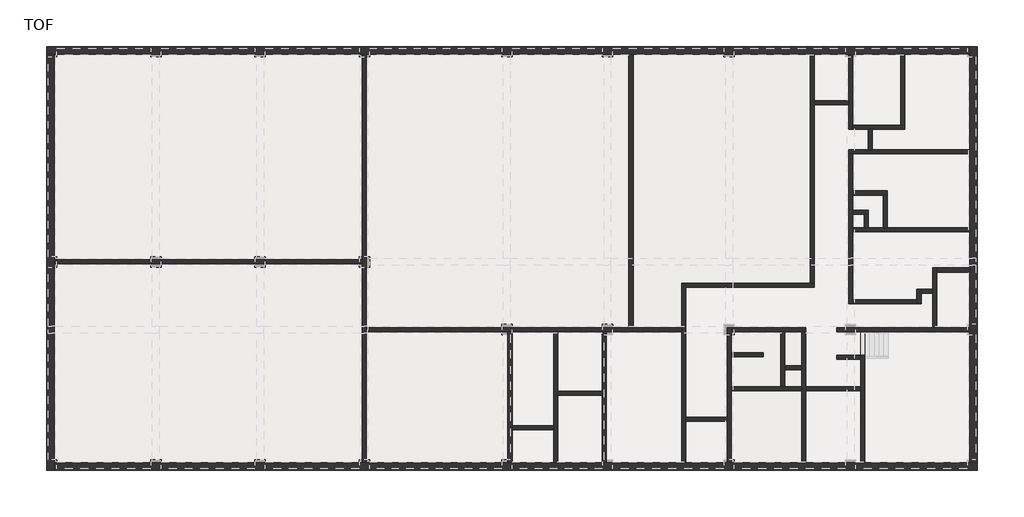
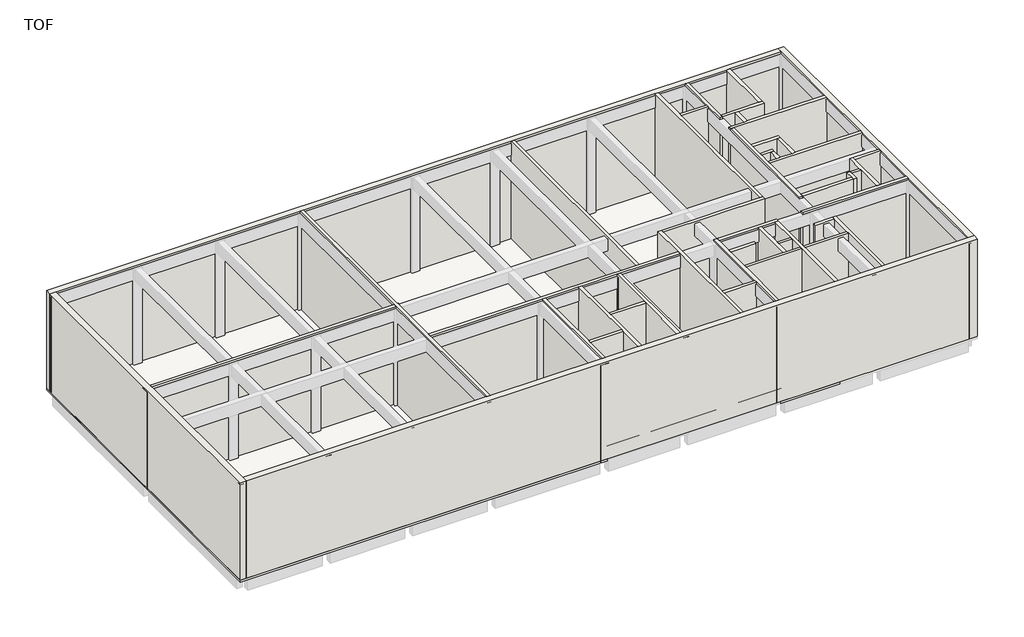
# One storey, part 1 of 3: 45 walls, 3 slabs.
"""IFC4 building model written with IfcOpenShell, lengths in millimetres."""

from ifc_helpers import new_model, si_unit, frame, origin, origin_with_axes, place, context, project, spatial, polyline, outline, extrude, faceted_brep, element, save

model = new_model("IFC4")

# Units and contexts
model_context = context("Model", 3, world=origin())
ifc_project = project(units=[si_unit("LENGTHUNIT", "METRE", prefix="MILLI")], contexts=[model_context])

# Site, building, storey
site = spatial("IfcSite", under=ifc_project)
building = spatial("IfcBuilding", under=site)
storey = spatial("IfcBuildingStorey", under=building, Name="TOF", Elevation=150.0)

# Slabs
placement = place(None, origin())
element("IfcSlab", 1, ObjectType="H_FL_AMF_RC Slab_T150", at=placement, inside=storey, context=model_context, shape_type="Brep", body=[
    faceted_brep([(-375.3, 24716.5208589, 0.0), (43724.7, 24716.5208589, 0.0), (43724.7, 10966.5208589, 0.0), (36324.7, 10966.5208589, 0.0), (36324.7, 8416.5208589, 0.0), (32224.7, 8416.5208589, 0.0), (31624.7, 8416.5208589, 0.0), (26424.7, 8416.5208589, 0.0), (25824.7, 8416.5208589, 0.0), (17924.7, 8416.5208589, 0.0), (17924.7, 12016.5208589, 0.0), (17924.7, 12316.5208589, 0.0), (17624.7, 12316.5208589, 0.0), (12224.7, 12316.5208589, 0.0), (11624.7, 12316.5208589, 0.0), (6224.7, 12316.5208589, 0.0), (5624.7, 12316.5208589, 0.0), (224.7, 12316.5208589, 0.0), (-375.3, 12316.5208589, 0.0), (-375.3, 24716.5208589, 150.0), (-375.3, 24116.5208589, 150.0), (-375.3, 12616.5208589, 150.0), (-375.3, 12316.5208589, 150.0), (224.7, 12316.5208589, 150.0), (5624.7, 12316.5208589, 150.0), (6224.7, 12316.5208589, 150.0), (11624.7, 12316.5208589, 150.0), (12224.7, 12316.5208589, 150.0), (17624.7, 12316.5208589, 150.0), (17924.7, 12316.5208589, 150.0), (17924.7, 12016.5208589, 150.0), (17924.7, 8416.5208589, 150.0), (25824.7, 8416.5208589, 150.0), (26424.7, 8416.5208589, 150.0), (31624.7, 8416.5208589, 150.0), (32224.7, 8416.5208589, 150.0), (36324.7, 8416.5208589, 150.0), (36324.7, 10966.5208589, 150.0), (43724.7, 10966.5208589, 150.0), (43724.7, 24716.5208589, 150.0), (39224.7, 24716.5208589, 150.0), (38624.7, 24716.5208589, 150.0), (32224.7, 24716.5208589, 150.0), (31624.7, 24716.5208589, 150.0), (26424.7, 24716.5208589, 150.0), (25824.7, 24716.5208589, 150.0), (18224.7, 24716.5208589, 150.0), (17624.7, 24716.5208589, 150.0), (12224.7, 24716.5208589, 150.0), (11624.7, 24716.5208589, 150.0), (6224.7, 24716.5208589, 150.0), (5624.7, 24716.5208589, 150.0), (224.7, 24716.5208589, 150.0)], [[[0, 1, 2, 3, 4, 5, 6, 7, 8, 9, 10, 11, 12, 13, 14, 15, 16, 17, 18]], [[19, 20, 21, 22, 23, 24, 25, 26, 27, 28, 29, 30, 31, 32, 33, 34, 35, 36, 37, 38, 39, 40, 41, 42, 43, 44, 45, 46, 47, 48, 49, 50, 51, 52]], [[0, 18, 22, 21, 20, 19]], [[1, 0, 19, 52, 51, 50, 49, 48, 47, 46, 45, 44, 43, 42, 41, 40, 39]], [[2, 1, 39, 38]], [[3, 2, 38, 37]], [[4, 3, 37, 36]], [[9, 8, 7, 6, 5, 4, 36, 35, 34, 33, 32, 31]], [[11, 10, 9, 31, 30, 29]], [[18, 17, 16, 15, 14, 13, 12, 11, 29, 28, 27, 26, 25, 24, 23, 22]]]),
])
element("IfcSlab", 2, ObjectType="H_FL_AMF_RC Slab_T150", at=placement, inside=storey, context=model_context, shape_type="SweptSolid", body=[
    extrude(outline(polyline([(17924.7, 12316.5208589), (17924.7, 8416.5208589), (26307.7, 8416.5208589), (26307.7, 316.5208589), (-375.3, 316.5208589), (-375.3, 12316.5208589), (17924.7, 12316.5208589)])), origin_with_axes(), (0.0, 0.0, 1.0), 150.0),
])
element("IfcSlab", 3, ObjectType="H_FL_AMF_RC Slab_T150", at=placement, inside=storey, context=model_context, shape_type="SweptSolid", body=[
    extrude(outline(polyline([(38924.7, 316.5208589), (38924.7, 8416.5208589), (43224.7, 8416.5208589), (43224.7, 316.5208589), (38924.7, 316.5208589)])), origin_with_axes(), (0.0, 0.0, 1.0), 150.0),
])

# Walls
element("IfcWall", 4, ObjectType="H_WA_AMW_Brick Wall_Ext (0.5B_50_1.0B / Emulsion)", at=placement, inside=storey, context=model_context, shape_type="Brep", body=[
    faceted_brep([(-375.3, 24286.5208589, 150.0), (54.7, 24286.5208589, 150.0), (17807.7, 24286.5208589, 150.0), (18041.7, 24286.5208589, 150.0), (33157.7, 24286.5208589, 150.0), (33391.7, 24286.5208589, 150.0), (43607.7, 24286.5208589, 150.0), (43841.7, 24286.5208589, 150.0), (52794.7, 24286.5208589, 150.0), (52794.7, 24286.5208589, 7650.0), (49041.7, 24286.5208589, 7650.0), (48807.7, 24286.5208589, 7650.0), (46041.7, 24286.5208589, 7650.0), (45807.7, 24286.5208589, 7650.0), (43841.7, 24286.5208589, 7650.0), (43607.7, 24286.5208589, 7650.0), (33391.7, 24286.5208589, 7650.0), (33157.7, 24286.5208589, 7650.0), (18041.7, 24286.5208589, 7650.0), (17807.7, 24286.5208589, 7650.0), (54.7, 24286.5208589, 7650.0), (-375.3, 24286.5208589, 7650.0), (-375.3, 24716.5208589, 150.0), (-375.3, 24716.5208589, 7650.0), (52794.7, 24716.5208589, 7650.0), (52794.7, 24716.5208589, 150.0)], [[[0, 1, 2, 3, 4, 5, 6, 7, 8, 9, 10, 11, 12, 13, 14, 15, 16, 17, 18, 19, 20, 21]], [[22, 23, 24, 25]], [[8, 7, 6, 5, 4, 3, 2, 1, 0, 22, 25]], [[21, 20, 19, 18, 17, 16, 15, 14, 13, 12, 11, 10, 9, 24, 23]], [[0, 21, 23, 22]], [[9, 8, 25, 24]]]),
])
element("IfcWall", 5, ObjectType="H_WA_AMW_Brick Wall_Ext (0.5B_50_1.0B / Emulsion)", at=placement, inside=storey, context=model_context, shape_type="Brep", body=[
    faceted_brep([(54.7, 316.5208589, 150.0), (54.7, 746.5208589, 150.0), (54.7, 12199.5208589, 150.0), (54.7, 12433.5208589, 150.0), (54.7, 24286.5208589, 150.0), (54.7, 24286.5208589, 7650.0), (54.7, 12433.5208589, 7650.0), (54.7, 12199.5208589, 7650.0), (54.7, 746.5208589, 7650.0), (54.7, 316.5208589, 7650.0), (-375.3, 316.5208589, 150.0), (-375.3, 316.5208589, 7650.0), (-375.3, 24286.5208589, 7650.0), (-375.3, 24286.5208589, 150.0)], [[[0, 1, 2, 3, 4, 5, 6, 7, 8, 9]], [[10, 11, 12, 13]], [[4, 3, 2, 1, 0, 10, 13]], [[9, 8, 7, 6, 5, 12, 11]], [[0, 9, 11, 10]], [[5, 4, 13, 12]]]),
])
element("IfcWall", 6, ObjectType="H_WA_AMW_Brick Wall_Ext (0.5B_50_1.0B / Emulsion)", at=placement, inside=storey, context=model_context, shape_type="Brep", body=[
    faceted_brep([(53224.7, 746.5208589, 150.0), (52794.7, 746.5208589, 150.0), (46741.7, 746.5208589, 150.0), (46507.7, 746.5208589, 150.0), (43341.7, 746.5208589, 150.0), (43107.7, 746.5208589, 150.0), (39041.7, 746.5208589, 150.0), (38807.7, 746.5208589, 150.0), (26424.7, 746.5208589, 150.0), (26190.7, 746.5208589, 150.0), (18041.7, 746.5208589, 150.0), (17807.7, 746.5208589, 150.0), (54.7, 746.5208589, 150.0), (54.7, 746.5208589, 7650.0), (17807.7, 746.5208589, 7650.0), (18041.7, 746.5208589, 7650.0), (26190.7, 746.5208589, 7650.0), (26424.7, 746.5208589, 7650.0), (28824.7, 746.5208589, 7650.0), (29058.7, 746.5208589, 7650.0), (31624.7, 746.5208589, 7650.0), (31858.7, 746.5208589, 7650.0), (36207.7, 746.5208589, 7650.0), (36441.7, 746.5208589, 7650.0), (38807.7, 746.5208589, 7650.0), (39041.7, 746.5208589, 7650.0), (43107.7, 746.5208589, 7650.0), (43341.7, 746.5208589, 7650.0), (46507.7, 746.5208589, 7650.0), (46741.7, 746.5208589, 7650.0), (52794.7, 746.5208589, 7650.0), (53224.7, 746.5208589, 7650.0), (53224.7, 316.5208589, 150.0), (53224.7, 316.5208589, 7650.0), (54.7, 316.5208589, 7650.0), (54.7, 316.5208589, 150.0)], [[[0, 1, 2, 3, 4, 5, 6, 7, 8, 9, 10, 11, 12, 13, 14, 15, 16, 17, 18, 19, 20, 21, 22, 23, 24, 25, 26, 27, 28, 29, 30, 31]], [[32, 33, 34, 35]], [[12, 11, 10, 9, 8, 7, 6, 5, 4, 3, 2, 1, 0, 32, 35]], [[31, 30, 29, 28, 27, 26, 25, 24, 23, 22, 21, 20, 19, 18, 17, 16, 15, 14, 13, 34, 33]], [[0, 31, 33, 32]], [[13, 12, 35, 34]]]),
])
element("IfcWall", 7, ObjectType="H_WA_AMW_Brick Wall_Ext (0.5B_50_1.0B / Emulsion)", at=placement, inside=storey, context=model_context, shape_type="Brep", body=[
    faceted_brep([(52794.7, 24716.5208589, 150.0), (52794.7, 24286.5208589, 150.0), (52794.7, 8533.5208589, 150.0), (52794.7, 8299.5208589, 150.0), (52794.7, 746.5208589, 150.0), (52794.7, 746.5208589, 7650.0), (52794.7, 8299.5208589, 7650.0), (52794.7, 8533.5208589, 7650.0), (52794.7, 11733.5208589, 7650.0), (52794.7, 11967.5208589, 7650.0), (52794.7, 14049.5208589, 7650.0), (52794.7, 14283.5208589, 7650.0), (52794.7, 18549.5208589, 7650.0), (52794.7, 18783.5208589, 7650.0), (52794.7, 24286.5208589, 7650.0), (52794.7, 24716.5208589, 7650.0), (53224.7, 24716.5208589, 150.0), (53224.7, 24716.5208589, 7650.0), (53224.7, 746.5208589, 7650.0), (53224.7, 746.5208589, 150.0)], [[[0, 1, 2, 3, 4, 5, 6, 7, 8, 9, 10, 11, 12, 13, 14, 15]], [[16, 17, 18, 19]], [[4, 3, 2, 1, 0, 16, 19]], [[15, 14, 13, 12, 11, 10, 9, 8, 7, 6, 5, 18, 17]], [[0, 15, 17, 16]], [[5, 4, 19, 18]]]),
])
element("IfcWall", 8, ObjectType="H_WA_AMW_Block Wall_Int_T200 (Both Plaster_Emulsion)", at=placement, inside=storey, context=model_context, shape_type="SweptSolid", body=[
    extrude(outline(polyline([(17807.7, 12199.5208589), (54.7, 12199.5208589), (54.7, 12433.5208589), (17807.7, 12433.5208589), (17807.7, 12199.5208589)])), frame((0.0, 0.0, 150.0), z_axis=(0.0, 0.0, 1.0), x_axis=(1.0, 0.0, 0.0)), (0.0, 0.0, 1.0), 7500.0),
])
element("IfcWall", 9, ObjectType="H_WA_AMW_Block Wall_Int_T200 (Both Plaster_Emulsion)", at=placement, inside=storey, context=model_context, shape_type="Brep", body=[
    faceted_brep([(17807.7, 24286.5208589, 150.0), (17807.7, 12433.5208589, 150.0), (17807.7, 12199.5208589, 150.0), (17807.7, 746.5208589, 150.0), (17807.7, 746.5208589, 7650.0), (17807.7, 12199.5208589, 7650.0), (17807.7, 12433.5208589, 7650.0), (17807.7, 24286.5208589, 7650.0), (18041.7, 24286.5208589, 150.0), (18041.7, 24286.5208589, 7650.0), (18041.7, 8533.5208589, 7650.0), (18041.7, 8299.5208589, 7650.0), (18041.7, 746.5208589, 7650.0), (18041.7, 746.5208589, 150.0), (18041.7, 8299.5208589, 150.0), (18041.7, 8533.5208589, 150.0)], [[[0, 1, 2, 3, 4, 5, 6, 7]], [[8, 9, 10, 11, 12, 13, 14, 15]], [[3, 2, 1, 0, 8, 15, 14, 13]], [[7, 6, 5, 4, 12, 11, 10, 9]], [[0, 7, 9, 8]], [[4, 3, 13, 12]]]),
])
element("IfcWall", 10, ObjectType="H_WA_AMW_Block Wall_Int_T200 (Both Plaster_Emulsion)", at=placement, inside=storey, context=model_context, shape_type="SweptSolid", body=[
    extrude(outline(polyline([(33157.7, 8533.5208589), (33157.7, 24286.5208589), (33391.7, 24286.5208589), (33391.7, 8533.5208589), (33157.7, 8533.5208589)])), frame((0.0, 0.0, 150.0), z_axis=(0.0, 0.0, 1.0), x_axis=(1.0, 0.0, 0.0)), (0.0, 0.0, 1.0), 7500.0),
])
element("IfcWall", 11, ObjectType="H_WA_AMW_Block Wall_Int_T200 (Both Plaster_Emulsion)", at=placement, inside=storey, context=model_context, shape_type="Brep", body=[
    faceted_brep([(18041.7, 8299.5208589, 150.0), (26190.7, 8299.5208589, 150.0), (26424.7, 8299.5208589, 150.0), (36207.7, 8299.5208589, 150.0), (36207.7, 8299.5208589, 7650.0), (31858.7, 8299.5208589, 7650.0), (31624.7, 8299.5208589, 7650.0), (29058.7, 8299.5208589, 7650.0), (28824.7, 8299.5208589, 7650.0), (26424.7, 8299.5208589, 7650.0), (26190.7, 8299.5208589, 7650.0), (18041.7, 8299.5208589, 7650.0), (18041.7, 8533.5208589, 150.0), (18041.7, 8533.5208589, 7650.0), (33157.7, 8533.5208589, 7650.0), (33391.7, 8533.5208589, 7650.0), (36207.7, 8533.5208589, 7650.0), (36207.7, 8533.5208589, 150.0), (33391.7, 8533.5208589, 150.0), (33157.7, 8533.5208589, 150.0)], [[[0, 1, 2, 3, 4, 5, 6, 7, 8, 9, 10, 11]], [[12, 13, 14, 15, 16, 17, 18, 19]], [[3, 2, 1, 0, 12, 19, 18, 17]], [[11, 10, 9, 8, 7, 6, 5, 4, 16, 15, 14, 13]], [[0, 11, 13, 12]], [[4, 3, 17, 16]]]),
])
element("IfcWall", 12, ObjectType="H_WA_AMW_Block Wall_Int_T200 (Both Plaster_Emulsion)", at=placement, inside=storey, context=model_context, shape_type="Brep", body=[
    faceted_brep([(36207.7, 11083.5208589, 1150.0), (36207.7, 746.5208589, 1150.0), (36207.7, 746.5208589, 7650.0), (36207.7, 8299.5208589, 7650.0), (36207.7, 8533.5208589, 7650.0), (36207.7, 11083.5208589, 7650.0), (36441.7, 11083.5208589, 1150.0), (36441.7, 11083.5208589, 7650.0), (36441.7, 10849.5208589, 7650.0), (36441.7, 3380.5208589, 7650.0), (36441.7, 3146.5208589, 7650.0), (36441.7, 746.5208589, 7650.0), (36441.7, 746.5208589, 1150.0), (36441.7, 3146.5208589, 1150.0), (36441.7, 3380.5208589, 1150.0)], [[[0, 1, 2, 3, 4, 5]], [[6, 7, 8, 9, 10, 11, 12, 13, 14]], [[1, 0, 6, 14, 13, 12]], [[5, 4, 3, 2, 11, 10, 9, 8, 7]], [[2, 1, 12, 11]], [[0, 5, 7, 6]]]),
])
element("IfcWall", 13, ObjectType="H_WA_AMW_Block Wall_Int_T200 (Both Plaster_Emulsion)", at=placement, inside=storey, context=model_context, shape_type="Brep", body=[
    faceted_brep([(36441.7, 10849.5208589, 150.0), (43841.7, 10849.5208589, 150.0), (43841.7, 10849.5208589, 7650.0), (36441.7, 10849.5208589, 7650.0), (36441.7, 11083.5208589, 150.0), (36441.7, 11083.5208589, 1150.0), (36441.7, 11083.5208589, 7650.0), (43607.7, 11083.5208589, 7650.0), (43841.7, 11083.5208589, 7650.0), (43841.7, 11083.5208589, 150.0), (43607.7, 11083.5208589, 150.0)], [[[0, 1, 2, 3]], [[4, 5, 6, 7, 8, 9, 10]], [[1, 0, 4, 10, 9]], [[3, 2, 8, 7, 6]], [[0, 3, 6, 5, 4]], [[2, 1, 9, 8]]]),
])
element("IfcWall", 14, ObjectType="H_WA_AMW_Block Wall_Int_T200 (Both Plaster_Emulsion)", at=placement, inside=storey, context=model_context, shape_type="Brep", body=[
    faceted_brep([(43841.7, 11083.5208589, 150.0), (43841.7, 24286.5208589, 150.0), (43841.7, 24286.5208589, 7650.0), (43841.7, 21586.5208589, 7650.0), (43841.7, 21352.5208589, 7650.0), (43841.7, 11083.5208589, 7650.0), (43607.7, 11083.5208589, 150.0), (43607.7, 11083.5208589, 7650.0), (43607.7, 24286.5208589, 7650.0), (43607.7, 24286.5208589, 150.0)], [[[0, 1, 2, 3, 4, 5]], [[6, 7, 8, 9]], [[1, 0, 6, 9]], [[5, 4, 3, 2, 8, 7]], [[0, 5, 7, 6]], [[2, 1, 9, 8]]]),
])
element("IfcWall", 15, ObjectType="H_WA_AMW_Block Wall_Int_T200 (Both Plaster_Emulsion)", at=placement, inside=storey, context=model_context, shape_type="SweptSolid", body=[
    extrude(outline(polyline([(45807.7, 21352.5208589), (43841.7, 21352.5208589), (43841.7, 21586.5208589), (45807.7, 21586.5208589), (45807.7, 21352.5208589)])), frame((0.0, 0.0, 1150.0), z_axis=(0.0, 0.0, 1.0), x_axis=(1.0, 0.0, 0.0)), (0.0, 0.0, 1.0), 6500.0),
])
element("IfcWall", 16, ObjectType="H_WA_AMW_Block Wall_Int_T200 (Both Plaster_Emulsion)", at=placement, inside=storey, context=model_context, shape_type="Brep", body=[
    faceted_brep([(45807.7, 24286.5208589, 1150.0), (45807.7, 21586.5208589, 1150.0), (45807.7, 21352.5208589, 1150.0), (45807.7, 19949.5208589, 1150.0), (45807.7, 19949.5208589, 7650.0), (45807.7, 21352.5208589, 7650.0), (45807.7, 21586.5208589, 7650.0), (45807.7, 24286.5208589, 7650.0), (46041.7, 24286.5208589, 1150.0), (46041.7, 24286.5208589, 7650.0), (46041.7, 20183.5208589, 7650.0), (46041.7, 19949.5208589, 7650.0), (46041.7, 19949.5208589, 1150.0), (46041.7, 20183.5208589, 1150.0)], [[[0, 1, 2, 3, 4, 5, 6, 7]], [[8, 9, 10, 11, 12, 13]], [[3, 2, 1, 0, 8, 13, 12]], [[7, 6, 5, 4, 11, 10, 9]], [[0, 7, 9, 8]], [[4, 3, 12, 11]]]),
])
element("IfcWall", 17, ObjectType="H_WA_AMW_Block Wall_Int_T200 (Both Plaster_Emulsion)", at=placement, inside=storey, context=model_context, shape_type="SweptSolid", body=[
    extrude(outline(polyline([(49743.7, 9899.5208589), (46041.7, 9899.5208589), (46041.7, 10133.5208589), (49743.7, 10133.5208589), (49743.7, 9899.5208589)])), frame((0.0, 0.0, 1150.0), z_axis=(0.0, 0.0, 1.0), x_axis=(1.0, 0.0, 0.0)), (0.0, 0.0, 1.0), 6500.0),
])
element("IfcWall", 18, ObjectType="H_WA_AMW_Block Wall_Int_T200 (Both Plaster_Emulsion)", at=placement, inside=storey, context=model_context, shape_type="Brep", body=[
    faceted_brep([(50660.7, 11967.5208589, 150.0), (50660.7, 8533.5208589, 150.0), (50660.7, 8533.5208589, 7650.0), (50660.7, 10499.5208589, 7650.0), (50660.7, 10733.5208589, 7650.0), (50660.7, 11967.5208589, 7650.0), (50894.7, 11967.5208589, 150.0), (50894.7, 11967.5208589, 1150.0), (50894.7, 11967.5208589, 7650.0), (50894.7, 11733.5208589, 7650.0), (50894.7, 8533.5208589, 7650.0), (50894.7, 8533.5208589, 150.0)], [[[0, 1, 2, 3, 4, 5]], [[6, 7, 8, 9, 10, 11]], [[1, 0, 6, 11]], [[5, 4, 3, 2, 10, 9, 8]], [[0, 5, 8, 7, 6]], [[2, 1, 11, 10]]]),
])
element("IfcWall", 19, ObjectType="H_WA_AMW_Block Wall_Int_T200 (Both Plaster_Emulsion)", at=placement, inside=storey, context=model_context, shape_type="SweptSolid", body=[
    extrude(outline(polyline([(52794.7, 11733.5208589), (50894.7, 11733.5208589), (50894.7, 11967.5208589), (52794.7, 11967.5208589), (52794.7, 11733.5208589)])), frame((0.0, 0.0, 1150.0), z_axis=(0.0, 0.0, 1.0), x_axis=(1.0, 0.0, 0.0)), (0.0, 0.0, 1.0), 6500.0),
])
element("IfcWall", 20, ObjectType="H_WA_AMW_Block Wall_Int_T200 (Both Plaster_Emulsion)", at=placement, inside=storey, context=model_context, shape_type="Brep", body=[
    faceted_brep([(49977.7, 9899.5208589, 1150.0), (49977.7, 10499.5208589, 1150.0), (49977.7, 10733.5208589, 1150.0), (49977.7, 10733.5208589, 7650.0), (49977.7, 10499.5208589, 7650.0), (49977.7, 9899.5208589, 7650.0), (49743.7, 9899.5208589, 1150.0), (49743.7, 9899.5208589, 7650.0), (49743.7, 10133.5208589, 7650.0), (49743.7, 10733.5208589, 7650.0), (49743.7, 10733.5208589, 1150.0), (49743.7, 10133.5208589, 1150.0)], [[[0, 1, 2, 3, 4, 5]], [[6, 7, 8, 9, 10, 11]], [[2, 1, 0, 6, 11, 10]], [[5, 4, 3, 9, 8, 7]], [[3, 2, 10, 9]], [[0, 5, 7, 6]]]),
])
element("IfcWall", 21, ObjectType="H_WA_AMW_Block Wall_Int_T200 (Both Plaster_Emulsion)", at=placement, inside=storey, context=model_context, shape_type="SweptSolid", body=[
    extrude(outline(polyline([(50660.7, 10499.5208589), (49977.7, 10499.5208589), (49977.7, 10733.5208589), (50660.7, 10733.5208589), (50660.7, 10499.5208589)])), frame((0.0, 0.0, 1150.0), z_axis=(0.0, 0.0, 1.0), x_axis=(1.0, 0.0, 0.0)), (0.0, 0.0, 1.0), 6500.0),
])
element("IfcWall", 22, ObjectType="H_WA_AMW_Block Wall_Int_T200 (Both Plaster_Emulsion)", at=placement, inside=storey, context=model_context, shape_type="Brep", body=[
    faceted_brep([(46507.7, 6933.5208589, 7650.0), (46507.7, 6933.5208589, 1150.0), (46507.7, 6933.5208589, 150.0), (46507.7, 6699.5208589, 150.0), (46507.7, 5130.5208589, 150.0), (46507.7, 4896.5208589, 150.0), (46507.7, 746.5208589, 150.0), (46507.7, 746.5208589, 7650.0), (46507.7, 4896.5208589, 7650.0), (46507.7, 5130.5208589, 7650.0), (46507.7, 6699.5208589, 7650.0), (46741.7, 6933.5208589, 150.0), (46741.7, 6933.5208589, 1150.0), (46741.7, 6933.5208589, 7650.0), (46741.7, 746.5208589, 7650.0), (46741.7, 746.5208589, 150.0)], [[[0, 1, 2, 3, 4, 5, 6, 7, 8, 9, 10]], [[11, 12, 13, 14, 15]], [[6, 5, 4, 3, 2, 11, 15]], [[0, 10, 9, 8, 7, 14, 13]], [[7, 6, 15, 14]], [[0, 13, 12, 11, 2, 1]]]),
])
element("IfcWall", 23, ObjectType="H_WA_AMW_Block Wall_Int_T200 (Both Plaster_Emulsion)", at=placement, inside=storey, context=model_context, shape_type="SweptSolid", body=[
    extrude(outline(polyline([(46507.7, 6699.5208589), (45124.7, 6699.5208589), (45124.7, 6933.5208589), (46507.7, 6933.5208589), (46507.7, 6699.5208589)])), frame((0.0, 0.0, 150.0), z_axis=(0.0, 0.0, 1.0), x_axis=(1.0, 0.0, 0.0)), (0.0, 0.0, 1.0), 7500.0),
])
element("IfcWall", 24, ObjectType="H_WA_AMW_Block Wall_Int_T200 (Both Plaster_Emulsion)", at=placement, inside=storey, context=model_context, shape_type="Brep", body=[
    faceted_brep([(52794.7, 8533.5208589, 150.0), (50894.7, 8533.5208589, 150.0), (50660.7, 8533.5208589, 150.0), (45124.7, 8533.5208589, 150.0), (45124.7, 8533.5208589, 7650.0), (50660.7, 8533.5208589, 7650.0), (50894.7, 8533.5208589, 7650.0), (52794.7, 8533.5208589, 7650.0), (52794.7, 8299.5208589, 150.0), (52794.7, 8299.5208589, 7650.0), (45124.7, 8299.5208589, 7650.0), (45124.7, 8299.5208589, 150.0), (46507.7, 8299.5208589, 150.0), (46741.7, 8299.5208589, 150.0)], [[[0, 1, 2, 3, 4, 5, 6, 7]], [[8, 9, 10, 11, 12, 13]], [[3, 2, 1, 0, 8, 13, 12, 11]], [[4, 3, 11, 10]], [[7, 6, 5, 4, 10, 9]], [[0, 7, 9, 8]]]),
])
element("IfcWall", 25, ObjectType="H_WA_AMW_Block Wall_Int_T200 (Both Plaster_Emulsion)", at=placement, inside=storey, context=model_context, shape_type="Brep", body=[
    faceted_brep([(38807.7, 8533.5208589, 150.0), (38807.7, 746.5208589, 150.0), (38807.7, 746.5208589, 1000.0), (38807.7, 8533.5208589, 1000.0), (38807.7, 746.5208589, 7650.0), (38807.7, 3146.5208589, 7650.0), (38807.7, 3380.5208589, 7650.0), (38807.7, 8533.5208589, 7650.0), (38807.7, 8533.5208589, 1150.0), (38807.7, 3380.5208589, 1150.0), (38807.7, 3146.5208589, 1150.0), (38807.7, 746.5208589, 1150.0), (39041.7, 746.5208589, 150.0), (39041.7, 4896.5208589, 150.0), (39041.7, 5130.5208589, 150.0), (39041.7, 6846.5208589, 150.0), (39041.7, 7080.5208589, 150.0), (39041.7, 8299.5208589, 150.0), (39041.7, 8533.5208589, 150.0), (39041.7, 8533.5208589, 1000.0), (39041.7, 8416.5208589, 1000.0), (39041.7, 8416.5208589, 1150.0), (39041.7, 8533.5208589, 1150.0), (39041.7, 8533.5208589, 7650.0), (39041.7, 8299.5208589, 7650.0), (39041.7, 7080.5208589, 7650.0), (39041.7, 6846.5208589, 7650.0), (39041.7, 5130.5208589, 7650.0), (39041.7, 4896.5208589, 7650.0), (39041.7, 746.5208589, 7650.0), (38924.7, 746.5208589, 1150.0), (38924.7, 746.5208589, 1000.0), (38924.7, 8416.5208589, 1000.0), (38924.7, 8416.5208589, 1150.0)], [[[0, 1, 2, 3]], [[4, 5, 6, 7, 8, 9, 10, 11]], [[12, 13, 14, 15, 16, 17, 18, 19, 20, 21, 22, 23, 24, 25, 26, 27, 28, 29]], [[1, 0, 18, 17, 16, 15, 14, 13, 12]], [[7, 6, 5, 4, 29, 28, 27, 26, 25, 24, 23]], [[1, 12, 29, 4, 11, 30, 31, 2]], [[7, 23, 22, 8]], [[18, 0, 3, 19]], [[31, 32, 20, 19, 3, 2]], [[21, 33, 30, 11, 10, 9, 8, 22]], [[32, 33, 21, 20]], [[33, 32, 31, 30]]]),
])
element("IfcWall", 26, ObjectType="H_WA_AMW_Block Wall_Int_T200 (Both Plaster_Emulsion)", at=placement, inside=storey, context=model_context, shape_type="Brep", body=[
    faceted_brep([(39041.7, 8299.5208589, 150.0), (41890.7, 8299.5208589, 150.0), (42124.7, 8299.5208589, 150.0), (43107.7, 8299.5208589, 150.0), (43341.7, 8299.5208589, 150.0), (43341.7, 8299.5208589, 1000.0), (43224.7, 8299.5208589, 1000.0), (43224.7, 8299.5208589, 1150.0), (43341.7, 8299.5208589, 1150.0), (43341.7, 8299.5208589, 7650.0), (43107.7, 8299.5208589, 7650.0), (42124.7, 8299.5208589, 7650.0), (41890.7, 8299.5208589, 7650.0), (39041.7, 8299.5208589, 7650.0), (43341.7, 8533.5208589, 150.0), (39041.7, 8533.5208589, 150.0), (39041.7, 8533.5208589, 1000.0), (43341.7, 8533.5208589, 1000.0), (39041.7, 8533.5208589, 7650.0), (43341.7, 8533.5208589, 7650.0), (43341.7, 8533.5208589, 1150.0), (39041.7, 8533.5208589, 1150.0), (39041.7, 8416.5208589, 1150.0), (39041.7, 8416.5208589, 1000.0), (43224.7, 8416.5208589, 1000.0), (43224.7, 8416.5208589, 1150.0)], [[[0, 1, 2, 3, 4, 5, 6, 7, 8, 9, 10, 11, 12, 13]], [[14, 15, 16, 17]], [[18, 19, 20, 21]], [[4, 3, 2, 1, 0, 15, 14]], [[13, 12, 11, 10, 9, 19, 18]], [[0, 13, 18, 21, 22, 23, 16, 15]], [[4, 14, 17, 5]], [[19, 9, 8, 20]], [[23, 24, 6, 5, 17, 16]], [[7, 25, 22, 21, 20, 8]], [[24, 25, 7, 6]], [[25, 24, 23, 22]]]),
])
element("IfcWall", 27, ObjectType="H_WA_AMW_Block Wall_Int_T200 (Both Plaster_Emulsion)", at=placement, inside=storey, context=model_context, shape_type="Brep", body=[
    faceted_brep([(43107.7, 8299.5208589, 150.0), (43107.7, 6333.5208589, 150.0), (43107.7, 6099.5208589, 150.0), (43107.7, 5130.5208589, 150.0), (43107.7, 4896.5208589, 150.0), (43107.7, 746.5208589, 150.0), (43107.7, 746.5208589, 7650.0), (43107.7, 4896.5208589, 7650.0), (43107.7, 5130.5208589, 7650.0), (43107.7, 6099.5208589, 7650.0), (43107.7, 6333.5208589, 7650.0), (43107.7, 8299.5208589, 7650.0), (43341.7, 746.5208589, 150.0), (43341.7, 4896.5208589, 150.0), (43341.7, 5130.5208589, 150.0), (43341.7, 8299.5208589, 150.0), (43341.7, 8299.5208589, 1000.0), (43341.7, 5013.5208589, 1000.0), (43341.7, 5013.5208589, 1150.0), (43341.7, 8299.5208589, 1150.0), (43341.7, 8299.5208589, 7650.0), (43341.7, 5130.5208589, 7650.0), (43341.7, 4896.5208589, 7650.0), (43341.7, 746.5208589, 7650.0), (43224.7, 8299.5208589, 1150.0), (43224.7, 8299.5208589, 1000.0), (43224.7, 5013.5208589, 1000.0), (43224.7, 5013.5208589, 1150.0)], [[[0, 1, 2, 3, 4, 5, 6, 7, 8, 9, 10, 11]], [[12, 13, 14, 15, 16, 17, 18, 19, 20, 21, 22, 23]], [[5, 4, 3, 2, 1, 0, 15, 14, 13, 12]], [[11, 10, 9, 8, 7, 6, 23, 22, 21, 20]], [[0, 11, 20, 19, 24, 25, 16, 15]], [[6, 5, 12, 23]], [[25, 26, 17, 16]], [[18, 27, 24, 19]], [[26, 27, 18, 17]], [[27, 26, 25, 24]]]),
])
element("IfcWall", 28, ObjectType="H_WA_AMW_Block Wall_Int_T200 (Both Plaster_Emulsion)", at=placement, inside=storey, context=model_context, shape_type="Brep", body=[
    faceted_brep([(39041.7, 4896.5208589, 7650.0), (39041.7, 4896.5208589, 150.0), (43107.7, 4896.5208589, 150.0), (43107.7, 4896.5208589, 7650.0), (39041.7, 5130.5208589, 150.0), (39041.7, 5130.5208589, 7650.0), (41890.7, 5130.5208589, 7650.0), (42124.7, 5130.5208589, 7650.0), (43107.7, 5130.5208589, 7650.0), (43107.7, 5130.5208589, 150.0), (42124.7, 5130.5208589, 150.0), (41890.7, 5130.5208589, 150.0)], [[[0, 1, 2, 3]], [[4, 5, 6, 7, 8, 9, 10, 11]], [[1, 4, 11, 10, 9, 2]], [[5, 0, 3, 8, 7, 6]], [[1, 0, 5, 4]], [[3, 2, 9, 8]]]),
    faceted_brep([(46507.7, 4896.5208589, 150.0), (46507.7, 4896.5208589, 7650.0), (43341.7, 4896.5208589, 7650.0), (43341.7, 4896.5208589, 150.0), (46507.7, 5130.5208589, 7650.0), (46507.7, 5130.5208589, 150.0), (43341.7, 5130.5208589, 150.0), (43341.7, 5130.5208589, 7650.0)], [[[0, 1, 2, 3]], [[4, 5, 6, 7]], [[5, 0, 3, 6]], [[1, 4, 7, 2]], [[1, 0, 5, 4]], [[3, 2, 7, 6]]]),
])
element("IfcWall", 29, ObjectType="H_WA_AMW_Block Wall_Int_T200 (Both Plaster_Emulsion)", at=placement, inside=storey, context=model_context, shape_type="SweptSolid", body=[
    extrude(outline(polyline([(40890.7, 6846.5208589), (39041.7, 6846.5208589), (39041.7, 7080.5208589), (40890.7, 7080.5208589), (40890.7, 6846.5208589)])), frame((0.0, 0.0, 150.0), z_axis=(0.0, 0.0, 1.0), x_axis=(1.0, 0.0, 0.0)), (0.0, 0.0, 1.0), 7500.0),
])
element("IfcWall", 30, ObjectType="H_WA_AMW_Block Wall_Int_T200 (Both Plaster_Emulsion)", at=placement, inside=storey, context=model_context, shape_type="Brep", body=[
    faceted_brep([(41890.7, 8299.5208589, 150.0), (41890.7, 5130.5208589, 150.0), (41890.7, 5130.5208589, 7650.0), (41890.7, 8299.5208589, 7650.0), (42124.7, 8299.5208589, 150.0), (42124.7, 8299.5208589, 7650.0), (42124.7, 6333.5208589, 7650.0), (42124.7, 6099.5208589, 7650.0), (42124.7, 5130.5208589, 7650.0), (42124.7, 5130.5208589, 150.0), (42124.7, 6099.5208589, 150.0), (42124.7, 6333.5208589, 150.0)], [[[0, 1, 2, 3]], [[4, 5, 6, 7, 8, 9, 10, 11]], [[1, 0, 4, 11, 10, 9]], [[3, 2, 8, 7, 6, 5]], [[0, 3, 5, 4]], [[2, 1, 9, 8]]]),
])
element("IfcWall", 31, ObjectType="H_WA_AMW_Block Wall_Int_T200 (Both Plaster_Emulsion)", at=placement, inside=storey, context=model_context, shape_type="SweptSolid", body=[
    extrude(outline(polyline([(43107.7, 6099.5208589), (42124.7, 6099.5208589), (42124.7, 6333.5208589), (43107.7, 6333.5208589), (43107.7, 6099.5208589)])), frame((0.0, 0.0, 150.0), z_axis=(0.0, 0.0, 1.0), x_axis=(1.0, 0.0, 0.0)), (0.0, 0.0, 1.0), 7500.0),
])
element("IfcWall", 32, ObjectType="H_WA_AMW_Block Wall_Int_T200 (Both Plaster_Emulsion)", at=placement, inside=storey, context=model_context, shape_type="Brep", body=[
    faceted_brep([(31624.7, 8299.5208589, 1150.0), (31624.7, 4880.5208589, 1150.0), (31624.7, 4646.5208589, 1150.0), (31624.7, 746.5208589, 1150.0), (31624.7, 746.5208589, 7650.0), (31624.7, 4646.5208589, 7650.0), (31624.7, 4880.5208589, 7650.0), (31624.7, 8299.5208589, 7650.0), (31858.7, 8299.5208589, 1150.0), (31858.7, 8299.5208589, 7650.0), (31858.7, 746.5208589, 7650.0), (31858.7, 746.5208589, 1150.0)], [[[0, 1, 2, 3, 4, 5, 6, 7]], [[8, 9, 10, 11]], [[3, 2, 1, 0, 8, 11]], [[7, 6, 5, 4, 10, 9]], [[0, 7, 9, 8]], [[4, 3, 11, 10]]]),
])
element("IfcWall", 33, ObjectType="H_WA_AMW_Block Wall_Int_T200 (Both Plaster_Emulsion)", at=placement, inside=storey, context=model_context, shape_type="Brep", body=[
    faceted_brep([(28824.7, 8299.5208589, 1150.0), (28824.7, 2880.5208589, 1150.0), (28824.7, 2646.5208589, 1150.0), (28824.7, 746.5208589, 1150.0), (28824.7, 746.5208589, 7650.0), (28824.7, 2646.5208589, 7650.0), (28824.7, 2880.5208589, 7650.0), (28824.7, 8299.5208589, 7650.0), (29058.7, 8299.5208589, 1150.0), (29058.7, 8299.5208589, 7650.0), (29058.7, 4880.5208589, 7650.0), (29058.7, 4646.5208589, 7650.0), (29058.7, 746.5208589, 7650.0), (29058.7, 746.5208589, 1150.0), (29058.7, 4646.5208589, 1150.0), (29058.7, 4880.5208589, 1150.0)], [[[0, 1, 2, 3, 4, 5, 6, 7]], [[8, 9, 10, 11, 12, 13, 14, 15]], [[3, 2, 1, 0, 8, 15, 14, 13]], [[7, 6, 5, 4, 12, 11, 10, 9]], [[4, 3, 13, 12]], [[0, 7, 9, 8]]]),
])
element("IfcWall", 34, ObjectType="H_WA_AMW_Block Wall_Int_T200 (Both Plaster_Emulsion)", at=placement, inside=storey, context=model_context, shape_type="Brep", body=[
    faceted_brep([(26190.7, 8299.5208589, 150.0), (26190.7, 746.5208589, 150.0), (26190.7, 746.5208589, 7650.0), (26190.7, 8299.5208589, 7650.0), (26424.7, 8299.5208589, 150.0), (26424.7, 8299.5208589, 7650.0), (26424.7, 2880.5208589, 7650.0), (26424.7, 2646.5208589, 7650.0), (26424.7, 746.5208589, 7650.0), (26424.7, 746.5208589, 150.0)], [[[0, 1, 2, 3]], [[4, 5, 6, 7, 8, 9]], [[1, 0, 4, 9]], [[3, 2, 8, 7, 6, 5]], [[2, 1, 9, 8]], [[0, 3, 5, 4]]]),
])
element("IfcWall", 35, ObjectType="H_WA_AMW_Block Wall_Int_T200 (Both Plaster_Emulsion)", at=placement, inside=storey, context=model_context, shape_type="SweptSolid", body=[
    extrude(outline(polyline([(31624.7, 4646.5208589), (29058.7, 4646.5208589), (29058.7, 4880.5208589), (31624.7, 4880.5208589), (31624.7, 4646.5208589)])), frame((0.0, 0.0, 1150.0), z_axis=(0.0, 0.0, 1.0), x_axis=(1.0, 0.0, 0.0)), (0.0, 0.0, 1.0), 6500.0),
])
element("IfcWall", 36, ObjectType="H_WA_AMW_Block Wall_Int_T200 (Both Plaster_Emulsion)", at=placement, inside=storey, context=model_context, shape_type="SweptSolid", body=[
    extrude(outline(polyline([(28824.7, 2646.5208589), (26424.7, 2646.5208589), (26424.7, 2880.5208589), (28824.7, 2880.5208589), (28824.7, 2646.5208589)])), frame((0.0, 0.0, 1150.0), z_axis=(0.0, 0.0, 1.0), x_axis=(1.0, 0.0, 0.0)), (0.0, 0.0, 1.0), 6500.0),
])
element("IfcWall", 37, ObjectType="H_WA_AMW_Block Wall_Int_T200 (Both Plaster_Emulsion)", at=placement, inside=storey, context=model_context, shape_type="Brep", body=[
    faceted_brep([(45807.7, 18549.5208589, 1150.0), (46041.7, 18549.5208589, 1150.0), (52794.7, 18549.5208589, 1150.0), (52794.7, 18549.5208589, 7650.0), (46041.7, 18549.5208589, 7650.0), (45807.7, 18549.5208589, 7650.0), (45807.7, 18783.5208589, 1150.0), (45807.7, 18783.5208589, 7650.0), (46924.7, 18783.5208589, 7650.0), (47158.7, 18783.5208589, 7650.0), (52794.7, 18783.5208589, 7650.0), (52794.7, 18783.5208589, 1150.0), (47158.7, 18783.5208589, 1150.0), (46924.7, 18783.5208589, 1150.0)], [[[0, 1, 2, 3, 4, 5]], [[6, 7, 8, 9, 10, 11, 12, 13]], [[2, 1, 0, 6, 13, 12, 11]], [[5, 4, 3, 10, 9, 8, 7]], [[3, 2, 11, 10]], [[0, 5, 7, 6]]]),
])
element("IfcWall", 38, ObjectType="H_WA_AMW_Block Wall_Int_T200 (Both Plaster_Emulsion)", at=placement, inside=storey, context=model_context, shape_type="SweptSolid", body=[
    extrude(outline(polyline([(38807.7, 3146.5208589), (36441.7, 3146.5208589), (36441.7, 3380.5208589), (38807.7, 3380.5208589), (38807.7, 3146.5208589)])), frame((0.0, 0.0, 1150.0), z_axis=(0.0, 0.0, 1.0), x_axis=(1.0, 0.0, 0.0)), (0.0, 0.0, 1.0), 6500.0),
])
element("IfcWall", 39, ObjectType="H_WA_AMW_Block Wall_Int_T200 (Both Plaster_Emulsion)", at=placement, inside=storey, context=model_context, shape_type="Brep", body=[
    faceted_brep([(46041.7, 19949.5208589, 1150.0), (46924.7, 19949.5208589, 1150.0), (47158.7, 19949.5208589, 1150.0), (49041.7, 19949.5208589, 1150.0), (49041.7, 19949.5208589, 7650.0), (47158.7, 19949.5208589, 7650.0), (46924.7, 19949.5208589, 7650.0), (46041.7, 19949.5208589, 7650.0), (46041.7, 20183.5208589, 1150.0), (46041.7, 20183.5208589, 7650.0), (48807.7, 20183.5208589, 7650.0), (49041.7, 20183.5208589, 7650.0), (49041.7, 20183.5208589, 1150.0), (48807.7, 20183.5208589, 1150.0)], [[[0, 1, 2, 3, 4, 5, 6, 7]], [[8, 9, 10, 11, 12, 13]], [[3, 2, 1, 0, 8, 13, 12]], [[7, 6, 5, 4, 11, 10, 9]], [[4, 3, 12, 11]], [[0, 7, 9, 8]]]),
])
element("IfcWall", 40, ObjectType="H_WA_AMW_Block Wall_Int_T200 (Both Plaster_Emulsion)", at=placement, inside=storey, context=model_context, shape_type="SweptSolid", body=[
    extrude(outline(polyline([(48807.7, 20183.5208589), (48807.7, 24286.5208589), (49041.7, 24286.5208589), (49041.7, 20183.5208589), (48807.7, 20183.5208589)])), frame((0.0, 0.0, 1150.0), z_axis=(0.0, 0.0, 1.0), x_axis=(1.0, 0.0, 0.0)), (0.0, 0.0, 1.0), 6500.0),
])
element("IfcWall", 41, ObjectType="H_WA_AMW_Block Wall_Int_T200 (Both Plaster_Emulsion)", at=placement, inside=storey, context=model_context, shape_type="Brep", body=[
    faceted_brep([(45807.7, 18549.5208589, 1150.0), (45807.7, 9899.5208589, 1150.0), (45807.7, 9899.5208589, 7650.0), (45807.7, 18549.5208589, 7650.0), (46041.7, 18549.5208589, 1150.0), (46041.7, 18549.5208589, 7650.0), (46041.7, 16400.5208589, 7650.0), (46041.7, 16166.5208589, 7650.0), (46041.7, 15300.5208589, 7650.0), (46041.7, 15066.5208589, 7650.0), (46041.7, 14283.5208589, 7650.0), (46041.7, 14049.5208589, 7650.0), (46041.7, 10133.5208589, 7650.0), (46041.7, 9899.5208589, 7650.0), (46041.7, 9899.5208589, 1150.0), (46041.7, 10133.5208589, 1150.0), (46041.7, 14049.5208589, 1150.0), (46041.7, 14283.5208589, 1150.0), (46041.7, 15066.5208589, 1150.0), (46041.7, 15300.5208589, 1150.0), (46041.7, 16166.5208589, 1150.0), (46041.7, 16400.5208589, 1150.0)], [[[0, 1, 2, 3]], [[4, 5, 6, 7, 8, 9, 10, 11, 12, 13, 14, 15, 16, 17, 18, 19, 20, 21]], [[1, 0, 4, 21, 20, 19, 18, 17, 16, 15, 14]], [[3, 2, 13, 12, 11, 10, 9, 8, 7, 6, 5]], [[2, 1, 14, 13]], [[0, 3, 5, 4]]]),
])
element("IfcWall", 42, ObjectType="H_WA_AMW_Block Wall_Int_T200 (Both Plaster_Emulsion)", at=placement, inside=storey, context=model_context, shape_type="SweptSolid", body=[
    extrude(outline(polyline([(46924.7, 18783.5208589), (46924.7, 19949.5208589), (47158.7, 19949.5208589), (47158.7, 18783.5208589), (46924.7, 18783.5208589)])), frame((0.0, 0.0, 1150.0), z_axis=(0.0, 0.0, 1.0), x_axis=(1.0, 0.0, 0.0)), (0.0, 0.0, 1.0), 6500.0),
])
element("IfcWall", 43, ObjectType="H_WA_AMW_Block Wall_Int_T200 (Both Plaster_Emulsion)", at=placement, inside=storey, context=model_context, shape_type="Brep", body=[
    faceted_brep([(46041.7, 14049.5208589, 1150.0), (52794.7, 14049.5208589, 1150.0), (52794.7, 14049.5208589, 7650.0), (46041.7, 14049.5208589, 7650.0), (46041.7, 14283.5208589, 1150.0), (46041.7, 14283.5208589, 7650.0), (46707.7, 14283.5208589, 7650.0), (46941.7, 14283.5208589, 7650.0), (47807.7, 14283.5208589, 7650.0), (48041.7, 14283.5208589, 7650.0), (52794.7, 14283.5208589, 7650.0), (52794.7, 14283.5208589, 1150.0), (48041.7, 14283.5208589, 1150.0), (47807.7, 14283.5208589, 1150.0), (46941.7, 14283.5208589, 1150.0), (46707.7, 14283.5208589, 1150.0)], [[[0, 1, 2, 3]], [[4, 5, 6, 7, 8, 9, 10, 11, 12, 13, 14, 15]], [[1, 0, 4, 15, 14, 13, 12, 11]], [[3, 2, 10, 9, 8, 7, 6, 5]], [[2, 1, 11, 10]], [[0, 3, 5, 4]]]),
])
element("IfcWall", 44, ObjectType="H_WA_AMW_Block Wall_Int_T200 (Both Plaster_Emulsion)", at=placement, inside=storey, context=model_context, shape_type="Brep", body=[
    faceted_brep([(46041.7, 16166.5208589, 1150.0), (47807.7, 16166.5208589, 1150.0), (48041.7, 16166.5208589, 1150.0), (48041.7, 16166.5208589, 7650.0), (47807.7, 16166.5208589, 7650.0), (46041.7, 16166.5208589, 7650.0), (46041.7, 16400.5208589, 1150.0), (46041.7, 16400.5208589, 7650.0), (48041.7, 16400.5208589, 7650.0), (48041.7, 16400.5208589, 1150.0)], [[[0, 1, 2, 3, 4, 5]], [[6, 7, 8, 9]], [[2, 1, 0, 6, 9]], [[5, 4, 3, 8, 7]], [[0, 5, 7, 6]], [[3, 2, 9, 8]]]),
])
element("IfcWall", 45, ObjectType="H_WA_AMW_Block Wall_Int_T200 (Both Plaster_Emulsion)", at=placement, inside=storey, context=model_context, shape_type="SweptSolid", body=[
    extrude(outline(polyline([(47807.7, 14283.5208589), (47807.7, 16166.5208589), (48041.7, 16166.5208589), (48041.7, 14283.5208589), (47807.7, 14283.5208589)])), frame((0.0, 0.0, 1150.0), z_axis=(0.0, 0.0, 1.0), x_axis=(1.0, 0.0, 0.0)), (0.0, 0.0, 1.0), 6500.0),
])
element("IfcWall", 46, ObjectType="H_WA_AMW_Block Wall_Int_T200 (Both Plaster_Emulsion)", at=placement, inside=storey, context=model_context, shape_type="Brep", body=[
    faceted_brep([(46041.7, 15066.5208589, 1150.0), (46707.7, 15066.5208589, 1150.0), (46941.7, 15066.5208589, 1150.0), (46941.7, 15066.5208589, 7650.0), (46707.7, 15066.5208589, 7650.0), (46041.7, 15066.5208589, 7650.0), (46041.7, 15300.5208589, 1150.0), (46041.7, 15300.5208589, 7650.0), (46941.7, 15300.5208589, 7650.0), (46941.7, 15300.5208589, 1150.0)], [[[0, 1, 2, 3, 4, 5]], [[6, 7, 8, 9]], [[2, 1, 0, 6, 9]], [[5, 4, 3, 8, 7]], [[0, 5, 7, 6]], [[3, 2, 9, 8]]]),
])
element("IfcWall", 47, ObjectType="H_WA_AMW_Block Wall_Int_T200 (Both Plaster_Emulsion)", at=placement, inside=storey, context=model_context, shape_type="SweptSolid", body=[
    extrude(outline(polyline([(46707.7, 14283.5208589), (46707.7, 15066.5208589), (46941.7, 15066.5208589), (46941.7, 14283.5208589), (46707.7, 14283.5208589)])), frame((0.0, 0.0, 1150.0), z_axis=(0.0, 0.0, 1.0), x_axis=(1.0, 0.0, 0.0)), (0.0, 0.0, 1.0), 6500.0),
])
element("IfcWall", 48, ObjectType="H_WA_AMW_Block Wall_Int_T200 (Both Plaster_Emulsion)", at=placement, inside=storey, context=model_context, shape_type="SweptSolid", body=[
    extrude(outline(polyline([(46507.7, 6933.5208589), (46507.7, 8299.5208589), (46741.7, 8299.5208589), (46741.7, 6933.5208589), (46507.7, 6933.5208589)])), frame((0.0, 0.0, 150.0), z_axis=(0.0, 0.0, 1.0), x_axis=(1.0, 0.0, 0.0)), (0.0, 0.0, 1.0), 1000.0),
])

save(model, "model.ifc")

# Revit data of these elements
# Project information
#   Project Status = "Project Status"
#   Client Name = "현대엔지니어링"
#   Project Address = "서울시 종로구 율곡로 75(계동)"
#   Project Number = "-"
# Grids (mm)
#   "Y1": line (-3935.398, 24416.521) -> (58968.688, 24416.521)
#   "X1": line (-75.3, 29394.337) -> (-75.3, -4379.638)
#   "X2": line (5924.7, 29394.337) -> (5924.7, -4379.638)
#   "Y3": line (-3935.398, 8416.521) -> (58968.688, 8416.521)
#   "Y4": line (-3935.398, 616.521) -> (58968.688, 616.521)
#   "X3": line (11924.7, 29394.337) -> (11924.7, -4379.638)
#   "X4": line (17924.7, 29394.337) -> (17924.7, -4379.638)
#   "X5": line (26124.7, 29394.337) -> (26124.7, -4379.638)
#   "X6": line (31924.7, 29394.337) -> (31924.7, -4379.638)
#   "X7": line (38924.7, 29394.337) -> (38924.7, -4379.638)
#   "X8": line (45924.7, 29394.337) -> (45924.7, -4379.638)
#   "X9": line (52924.7, 29394.337) -> (52924.7, -4379.638)
#   "X15": line (43724.7, 27041.858) -> (43724.7, 9156.488)
#   "X16": line (36324.7, 27041.858) -> (36324.7, 9156.488)
#   "X17": line (34685.051, 10966.521) -> (55094.626, 10966.521)
#   "X18": line (34685.051, 18666.521) -> (55094.626, 18666.521)
#   "Y2": line (-3935.398, 12316.521) -> (58968.688, 12316.521)
# Type "H_FL_AMF_RC Slab_T150"
#   Keynote = ""
#   Type Comments = ""
#   Description = ""
#   Function = 1
#   Layers, outside or top first: 0.150 m no material (function 1)
# Type "H_WA_AMW_Brick Wall_Ext (0.5B_50_1.0B / Emulsion)"
#   Type Comments = ""
#   Layers, outside or top first: 0.000 m no material (function 100); 0.020 m no material (function 2); 0.115 m no material (function 1); 0.050 m no material (function 3); 0.000 m no material (function 100); 0.230 m no material (function 1); 0.015 m no material (function 2); 0.000 m no material (function 100); 0.000 m no material (function 100)
# Type "H_WA_AMW_Block Wall_Int_T200 (Both Plaster_Emulsion)"
#   Type Comments = ""
#   Layers, outside or top first: 0.000 m no material (function 100); 0.012 m no material (function 2); 0.200 m no material (function 1); 0.012 m no material (function 2); 0.010 m no material (function 5)
# Element 1 (IfcSlab, "H_FL_AMF_RC Slab_T150")
#   Height Offset From Level = 0.000 m
#   Phase Created = New Construction
#   Materials on its faces: "Default Floor"
# Element 2 (IfcSlab, "H_FL_AMF_RC Slab_T150")
#   built-in parameter 1001955 = 1.5708 (stored number, unit not read)
#   Height Offset From Level = 0.000 m
#   Phase Created = New Construction
#   Materials on its faces: "Default Floor"
# Element 3 (IfcSlab, "H_FL_AMF_RC Slab_T150")
#   built-in parameter 1001955 = -1.5708 (stored number, unit not read)
#   Height Offset From Level = 0.000 m
#   Phase Created = New Construction
#   Materials on its faces: "Default Floor"
# Elements 4, 5, 6, 7 (IfcWall, "H_WA_AMW_Brick Wall_Ext (0.5B_50_1.0B / Emulsion)")
#   Top Offset = 0.000 m
#   Base Offset = 0.000 m
#   wall height = 7.500 m
#   Phase Created = New Construction
#   Base Constraint = TOF
#   Top Constraint = TOC
#   Materials on its faces: "Default Wall"
# Elements 8, 9, 10, 11, 13, 14, 18, 22, 23, 24, 25, 26, 27, 28, 29, 30, 31, 34 (IfcWall, "H_WA_AMW_Block Wall_Int_T200 (Both Plaster_Emulsion)")
#   Top Offset = 0.000 m
#   Base Offset = 0.000 m
#   wall height = 7.500 m
#   Phase Created = New Construction
#   Base Constraint = TOF
#   Top Constraint = TOC
#   Materials on its faces: "Default Wall"
# Elements 12, 15, 16, 17, 19, 20, 21, 32, 33, 35, 36, 37, 38, 39, 40, 41, 42, 43, 44, 45, 46, 47 (IfcWall, "H_WA_AMW_Block Wall_Int_T200 (Both Plaster_Emulsion)")
#   built-in parameter 1001111 = 1.000 m
#   Top Offset = 0.000 m
#   Base Offset = 1.000 m
#   wall height = 6.500 m
#   Phase Created = New Construction
#   Base Constraint = TOF
#   Top Constraint = TOC
#   Materials on its faces: "Default Wall"
# Element 48 (IfcWall, "H_WA_AMW_Block Wall_Int_T200 (Both Plaster_Emulsion)")
#   Top Offset = 0.000 m
#   Base Offset = 0.000 m
#   Unconnected Height = 1.000 m
#   wall height = 1.000 m
#   Phase Created = New Construction
#   Base Constraint = TOF
#   Materials on its faces: "Default Wall"
# Materials
#   "Default Floor": class "Miscellaneous", colour RGB 80 80 80, transparency 0
#   "Default Wall": class "Miscellaneous", colour RGB 80 80 80, transparency 0
